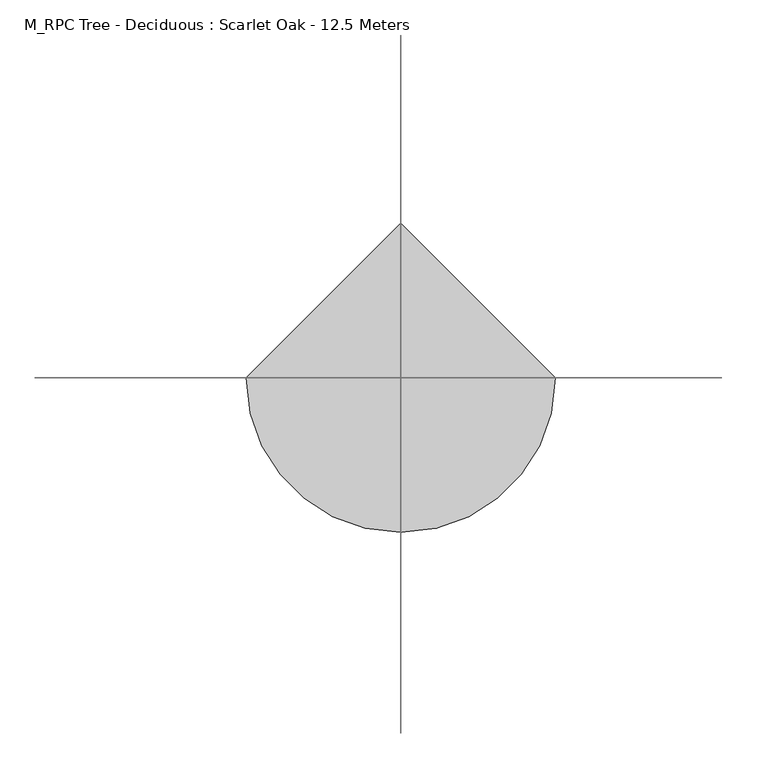
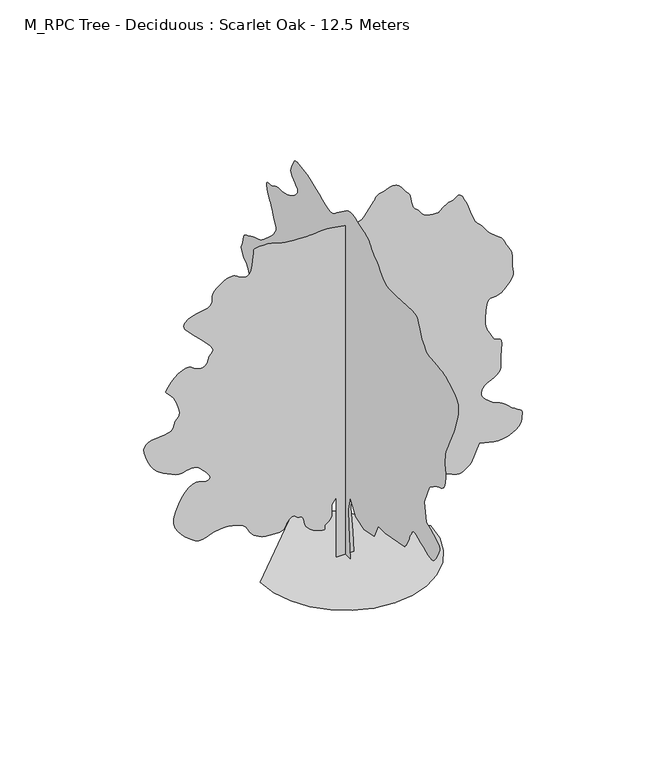
"""IFC4 building model written with IfcOpenShell, lengths in millimetres: geographic element geometry, M_RPC Tree - Deciduous : Scarlet Oak - 12.5 Meters."""

import ifcopenshell
import ifcopenshell.guid

model = None  # the IFC model being written
_history = None  # IfcOwnerHistory: only IFC2X3 demands one
_inside = {}  # id of a spatial element -> (the spatial element, [elements in it])
_under = {}  # id of a project, library or spatial element -> (it, [spatial elements below it])
_declared = {}  # id of a project -> (the project, [libraries it declares])
_typed = {}  # id of a type object -> (the type object, [elements of that type])
_made_of = {}  # id of a material, layer set ... -> (it, [elements and type objects made of it])


def new_model(schema):
    """Start an empty IFC model of exactly this schema.

    Asked for "IFC4X3", IfcOpenShell would pick the latest addendum, in which some entities
    have other attributes; the version numbers below select the first issue.
    IFC2X3 requires an IfcOwnerHistory on every rooted entity: one is made here for all.
    """
    global model, _history
    if schema == "IFC4X3":
        model = ifcopenshell.file(schema_version=(4, 3, 0, 0))
    else:
        model = ifcopenshell.file(schema=schema)
    _inside.clear()
    _under.clear()
    _declared.clear()
    _typed.clear()
    _made_of.clear()
    _history = None
    if model.schema == "IFC2X3":
        org = make("IfcOrganization", Name="unknown")
        user = make(
            "IfcPersonAndOrganization",
            ThePerson=make("IfcPerson", FamilyName="unknown"),
            TheOrganization=org,
        )
        app = make(
            "IfcApplication",
            ApplicationDeveloper=org,
            Version="unknown",
            ApplicationFullName="unknown",
            ApplicationIdentifier="unknown",
        )
        _history = make(
            "IfcOwnerHistory",
            OwningUser=user,
            OwningApplication=app,
            ChangeAction="ADDED",
            CreationDate=0,
        )
    return model


def make(cls, **values):
    """One entity of the class cls with the attributes given. An attribute that is None is left unset."""
    return model.create_entity(
        cls, **{name: value for name, value in values.items() if value is not None}
    )


def rooted(cls, **values):
    """An entity with a GlobalId (a new one), such as an element, a storey or a relation."""
    return make(cls, GlobalId=ifcopenshell.guid.new(), OwnerHistory=_history, **values)


def si_unit(unit_type, name, prefix=None):
    """IfcSIUnit, for example si_unit("LENGTHUNIT", "METRE", prefix="MILLI")."""
    return make("IfcSIUnit", UnitType=unit_type, Prefix=prefix, Name=name)


def assignment(units):
    """IfcUnitAssignment: the units of a project."""
    return None if units is None else make("IfcUnitAssignment", Units=units)


def point(xyz):
    """IfcCartesianPoint."""
    return None if xyz is None else make("IfcCartesianPoint", Coordinates=xyz)


def direction(xyz):
    """IfcDirection."""
    return None if xyz is None else make("IfcDirection", DirectionRatios=xyz)


def frame(location, z_axis=None, x_axis=None):
    """IfcAxis2Placement3D, a coordinate frame: its origin and axes. An axis left out is left unset."""
    return make(
        "IfcAxis2Placement3D",
        Location=point(location),
        Axis=direction(z_axis),
        RefDirection=direction(x_axis),
    )


def origin():
    """The frame at (0, 0, 0) with its axes left unset."""
    return frame((0.0, 0.0, 0.0))


def place(relative_to, where):
    """IfcLocalPlacement: puts the frame where relative to a parent placement (None: the world)."""
    return make(
        "IfcLocalPlacement", PlacementRelTo=relative_to, RelativePlacement=where
    )


def context(
    kind, dimensions, precision=None, world=None, true_north=None, identifier=None
):
    """IfcGeometricRepresentationContext, for example the 3D "Model" context."""
    return make(
        "IfcGeometricRepresentationContext",
        ContextIdentifier=identifier,
        ContextType=kind,
        CoordinateSpaceDimension=dimensions,
        Precision=precision,
        WorldCoordinateSystem=world,
        TrueNorth=true_north,
    )


def project(units=None, contexts=None):
    """IfcProject with its units and contexts."""
    return rooted(
        "IfcProject",
        Name="project",
        RepresentationContexts=contexts,
        UnitsInContext=assignment(units),
    )


def spatial(cls, under=None, at=None, **own):
    """A site, building, storey or space (cls), placed at a placement, below another one or the project."""
    s = rooted(cls, ObjectPlacement=at, **own)
    if under is not None:
        _under.setdefault(under.id(), (under, []))[1].append(s)
    return s


def point_list(points):
    """IfcCartesianPointList2D or 3D."""
    cls = (
        "IfcCartesianPointList2D" if len(points[0]) == 2 else "IfcCartesianPointList3D"
    )
    return make(cls, CoordList=points)


def triangles(points, corners, closed=None, point_numbers=None):
    """IfcTriangulatedFaceSet: each triangle names its three corners, points numbered from 1."""
    return make(
        "IfcTriangulatedFaceSet",
        Coordinates=point_list(points),
        Closed=closed,
        CoordIndex=corners,
        PnIndex=point_numbers,
    )


def shape(context_of_items, identifier, shape_type, items):
    """IfcShapeRepresentation: the items that make up one representation, for example the "Body"."""
    return make(
        "IfcShapeRepresentation",
        ContextOfItems=context_of_items,
        RepresentationIdentifier=identifier,
        RepresentationType=shape_type,
        Items=items,
    )


def source(mapping_origin, context_of_items, identifier, shape_type, items):
    """IfcRepresentationMap: a shape defined once, which mapped items show again and again."""
    return make(
        "IfcRepresentationMap",
        MappingOrigin=mapping_origin,
        MappedRepresentation=shape(context_of_items, identifier, shape_type, items),
    )


def transform(
    local_origin,
    x_axis=None,
    y_axis=None,
    z_axis=None,
    scale=None,
    scale2=None,
    scale3=None,
    uniform=True,
):
    """IfcCartesianTransformationOperator3D, or its non-uniform kind. x_axis, y_axis, z_axis: its Axis1, 2, 3."""
    if uniform:
        return make(
            "IfcCartesianTransformationOperator3D",
            Axis1=direction(x_axis),
            Axis2=direction(y_axis),
            LocalOrigin=point(local_origin),
            Scale=scale,
            Axis3=direction(z_axis),
        )
    return make(
        "IfcCartesianTransformationOperator3DnonUniform",
        Axis1=direction(x_axis),
        Axis2=direction(y_axis),
        LocalOrigin=point(local_origin),
        Scale=scale,
        Axis3=direction(z_axis),
        Scale2=scale2,
        Scale3=scale3,
    )


def mapped(mapping_source, mapping_target):
    """IfcMappedItem: shows the shape of a source again, moved by a transform."""
    return make(
        "IfcMappedItem", MappingSource=mapping_source, MappingTarget=mapping_target
    )


def made_of(thing, what):
    """Note that an element or type object is made of a material, layer set ...; save() writes the relation."""
    if what is not None:
        _made_of.setdefault(what.id(), (what, []))[1].append(thing)
    return thing


def element(
    cls,
    number,
    at=None,
    inside=None,
    cuts=None,
    type_object=None,
    material=None,
    context=None,
    identifier="Body",
    shape_type=None,
    held_by="IfcProductDefinitionShape",
    body=None,
    shapes=None,
    **own,
):
    """One element of the class cls, such as IfcWall. Its Tag is "e" and its number.

    at: its placement. inside: the storey or other place that contains it. cuts: it is an
    opening in that element (IfcRelVoidsElement). A single representation is given by context,
    identifier, shape_type and body (its items); several are given by shapes. held_by: the class
    of the entity that holds the representations. save() writes the other relations.
    """
    e = rooted(cls, Tag="e%d" % number, ObjectPlacement=at, **own)
    if body is not None:
        shapes = [shape(context, identifier, shape_type, body)]
    if shapes is not None:
        e.Representation = make(held_by, Representations=shapes)
    if inside is not None:
        _inside.setdefault(inside.id(), (inside, []))[1].append(e)
    if cuts is not None:
        rooted(
            "IfcRelVoidsElement", RelatingBuildingElement=cuts, RelatedOpeningElement=e
        )
    if type_object is not None:
        _typed.setdefault(type_object.id(), (type_object, []))[1].append(e)
    return made_of(e, material)


def aggregate(whole, parts):
    """IfcRelAggregates: a whole, such as a stair, and the parts it consists of."""
    return rooted("IfcRelAggregates", RelatingObject=whole, RelatedObjects=parts)


def save(model, path):
    """Write the relations noted so far, then the file.

    IfcRelAggregates (storeys below a building ...), IfcRelContainedInSpatialStructure (elements
    in a storey), IfcRelDefinesByType, IfcRelAssociatesMaterial and IfcRelDeclares: one each for
    every whole, place, type object, material and project.
    """
    for whole, parts in _under.values():
        aggregate(whole, parts)
    for where, things in _inside.values():
        rooted(
            "IfcRelContainedInSpatialStructure",
            RelatedElements=things,
            RelatingStructure=where,
        )
    for kind, things in _typed.values():
        rooted("IfcRelDefinesByType", RelatedObjects=things, RelatingType=kind)
    for what, things in _made_of.values():
        rooted("IfcRelAssociatesMaterial", RelatedObjects=things, RelatingMaterial=what)
    for by, libraries in _declared.values():
        rooted("IfcRelDeclares", RelatingContext=by, RelatedDefinitions=libraries)
    model.write(path)


def m_rpc_tree_deciduous_scarlet_oak_12_5_meters_13b38d7d(model_context):
    return source(origin(), model_context, "Body", "Tessellation", [
        triangles([(0.0172504, 306.0074844, 0.0), (0.0172504, -293.5650026, 0.0), (0.0172504, -196.8600042, 1141.1199549), (0.0172504, -177.5184886, 1682.6674953), (0.0172504, -293.5650026, 2185.5349113), (0.0172504, -603.0224945, 1682.6674953), (0.0172504, -1105.8875124, 1527.9400211), (0.0172504, -1686.1174301, 1663.3275421), (0.0172504, -1918.2099495, 2146.8525341), (0.0172504, -2324.3725124, 2146.8525341), (0.0172504, -3446.1498253, 2359.6049549), (0.0172504, -3487.4249222, 2409.394939), (0.0172504, -3527.7000801, 2459.5225479), (0.0172504, -3565.9250725, 2510.3249702), (0.0172504, -3601.0999603, 2562.1500046), (0.0172504, -3632.2248047, 2615.3249565), (0.0172504, -3658.2749588, 2670.2000954), (0.0172504, -3678.2499023, 2727.0748215), (0.0172504, -3697.649881, 2785.6750237), (0.0172504, -3722.1248405, 2845.2748741), (0.0172504, -3750.8248329, 2905.7249634), (0.0172504, -3782.89991, 2966.8500114), (0.0172504, -3817.5248314, 3028.475029), (0.0172504, -3853.8249413, 3090.4500252), (0.0172504, -3890.9999977, 3152.5750122), (0.0172504, -3908.7000801, 3172.6499496), (0.0172504, -3933.1750397, 3188.8498329), (0.0172504, -3971.1750458, 3197.2499016), (0.0172504, -4029.4749756, 3193.9748108), (0.0172504, -4114.8499969, 3175.1500877), (0.0172504, -4234.0499886, 3136.8498093), (0.0172504, -4393.8498276, 3075.2250824), (0.0172504, -4562.5749939, 3002.6998581), (0.0172504, -4706.2499451, 2937.9750298), (0.0172504, -4828.2750549, 2886.4249786), (0.0172504, -4932.0251175, 2853.4999535), (0.0172504, -5020.8999252, 2844.5999153), (0.0172504, -5098.249855, 2865.1248253), (0.0172504, -5167.4996979, 2920.4999336), (0.0172504, -5237.3750839, 3007.7248421), (0.0172504, -5309.5997452, 3113.9000473), (0.0172504, -5377.0996948, 3229.5499649), (0.0172504, -5432.7497864, 3345.1998825), (0.0172504, -5469.4498718, 3451.3750877), (0.0172504, -5480.1248016, 3538.6249947), (0.0172504, -5457.6250122, 3597.424894), (0.0172504, -5402.6498795, 3641.6998077), (0.0172504, -5323.3000717, 3691.0249947), (0.0172504, -5223.6747574, 3744.5999222), (0.0172504, -5107.774855, 3801.5499344), (0.0172504, -4979.7251129, 3861.0500816), (0.0172504, -4843.5499947, 3922.224836), (0.0172504, -4703.3248329, 3984.2498291), (0.0172504, -4587.2749397, 4641.8498062), (0.0172504, -4877.3749649, 5318.7747665), (0.0172504, -4886.5249878, 5331.7001404), (0.0172504, -4900.7247025, 5347.4747589), (0.0172504, -4925.0999588, 5369.0251877), (0.0172504, -4964.6748688, 5399.20009), (0.0172504, -5024.5497025, 5440.8498734), (0.0172504, -5109.8247299, 5496.8999405), (0.0172504, -5225.5246445, 5570.225116), (0.0172504, -5351.0501221, 5636.6501312), (0.0172504, -5462.3497238, 5680.0498077), (0.0172504, -5559.4501923, 5715.3499786), (0.0172504, -5642.3497833, 5757.424736), (0.0172504, -5711.0246613, 5821.1499161), (0.0172504, -5765.4998245, 5921.4001923), (0.0172504, -5805.7496933, 6073.0746552), (0.0172504, -5829.0500153, 6222.0498642), (0.0172504, -5835.7501877, 6317.5748474), (0.0172504, -5830.6249191, 6379.6001312), (0.0172504, -5818.3750854, 6428.1000778), (0.0172504, -5803.7748138, 6483.0246323), (0.0172504, -5791.5499786, 6564.3249023), (0.0172504, -5786.4247101, 6691.9996674), (0.0172504, -5788.2251816, 6832.849791), (0.0172504, -5796.1246994, 6949.6746368), (0.0172504, -5813.8247818, 7056.3751007), (0.0172504, -5845.0496201, 7166.7747574), (0.0172504, -5893.550148, 7294.7750839), (0.0172504, -5963.0249771, 7454.2496521), (0.0172504, -6057.1750443, 7659.049942), (0.0172504, -6146.5748199, 7844.1746887), (0.0172504, -6206.1746704, 7955.8748474), (0.0172504, -6246.4751175, 8024.9497009), (0.0172504, -6277.9999374, 8082.1746964), (0.0172504, -6311.2246536, 8158.3496979), (0.0172504, -6356.599791, 8284.2751511), (0.0172504, -6424.6747055, 8490.6997604), (0.0172504, -6498.0248795, 8729.4997192), (0.0172504, -6547.3747742, 8935.1499573), (0.0172504, -6565.2498459, 9112.3746048), (0.0172504, -6544.199968, 9265.925116), (0.0172504, -6476.8250107, 9400.5250397), (0.0172504, -6355.6498489, 9520.8996689), (0.0172504, -6173.2249374, 9631.8248749), (0.0172504, -5996.2246948, 9723.0001236), (0.0172504, -5879.7998245, 9785.7747803), (0.0172504, -5799.2250916, 9827.2001587), (0.0172504, -5729.799678, 9854.4496582), (0.0172504, -5646.85009, 9874.575174), (0.0172504, -5525.6749283, 9894.699527), (0.0172504, -5341.575119, 9921.9501892), (0.0172504, -5144.0999634, 9943.4244598), (0.0172504, -4990.9500092, 9951.725116), (0.0172504, -4869.5998581, 9962.0244873), (0.0172504, -4767.5499825, 9989.5995483), (0.0172504, -4672.2499855, 10049.6493713), (0.0172504, -4571.2000488, 10157.425351), (0.0172504, -4451.8750648, 10328.0998169), (0.0172504, -4347.6750298, 10515.7499908), (0.0172504, -4286.1000092, 10666.5500885), (0.0172504, -4245.8498497, 10783.8243256), (0.0172504, -4205.5749825, 10871.0003998), (0.0172504, -4143.9999619, 10931.4501984), (0.0172504, -4039.7999268, 10968.5502594), (0.0172504, -3871.650016, 10985.7003754), (0.0172504, -2943.2749969, 10927.6748474), (0.0172504, -2772.1499771, 10930.6746643), (0.0172504, -2632.8250511, 10930.2746887), (0.0172504, -2514.4500092, 10937.3242584), (0.0172504, -2406.244986, 10962.6250397), (0.0172504, -2297.3599171, 11017.0496246), (0.0172504, -2176.9724979, 11111.3752625), (0.0172504, -2034.2549011, 11256.4745453), (0.0172504, -1896.7275398, 11403.0249023), (0.0172504, -1793.7049038, 11502.8746216), (0.0172504, -1717.0749882, 11568.5752625), (0.0172504, -1658.7124168, 11612.6248993), (0.0172504, -1610.5024235, 11647.5250946), (0.0172504, -1564.3199226, 11685.7995026), (0.0172504, -1512.0500027, 11739.9996826), (0.0172504, -1461.8649845, 11803.9992645), (0.0172504, -1420.8125484, 11863.6002777), (0.0172504, -1379.087479, 11919.1503754), (0.0172504, -1326.8724976, 11970.9495392), (0.0172504, -1254.3574471, 12019.4000702), (0.0172504, -1151.7299904, 12064.7996246), (0.0172504, -1009.182514, 12107.4749268), (0.0172504, -849.1549999, 12154.4999634), (0.0172504, -699.9524792, 12206.6002716), (0.0172504, -560.5600064, 12254.6496643), (0.0172504, -429.9675053, 12289.4998627), (0.0172504, -307.1549798, 12302.0246796), (0.0172504, -191.1079934, 12283.0746735), (0.0172504, -80.8134993, 12223.5248199), (0.0172504, 499.4174812, 11798.0252106), (0.0172504, 562.2325061, 11740.8496307), (0.0172504, 623.0199657, 11688.7493225), (0.0172504, 689.217524, 11646.7751404), (0.0172504, 768.2749804, 11620.0500275), (0.0172504, 867.6299623, 11613.6248383), (0.0172504, 994.7275097, 11632.5748444), (0.0172504, 1157.0125168, 11681.9753174), (0.0172504, 1341.1749676, 11755.3243286), (0.0172504, 1526.6899521, 11837.8251068), (0.0172504, 1710.1749733, 11922.0246185), (0.0172504, 1888.2475342, 12000.4500641), (0.0172504, 2057.5249924, 12065.6995697), (0.0172504, 2214.6199093, 12110.3003357), (0.0172504, 2356.1550201, 12126.8249084), (0.0172504, 2484.8875694, 12135.849939), (0.0172504, 2604.4750374, 12156.3742676), (0.0172504, 2712.9248131, 12178.575238), (0.0172504, 2808.1498146, 12192.6743774), (0.0172504, 2888.1748718, 12188.8501923), (0.0172504, 2950.9248207, 12157.2753754), (0.0172504, 2994.400074, 12088.1249451), (0.0172504, 3033.2500282, 12001.2500153), (0.0172504, 3077.8499222, 11921.1246735), (0.0172504, 3119.7499809, 11845.0502472), (0.0172504, 3150.4998482, 11770.3245758), (0.0172504, 3161.6000427, 11694.2745667), (0.0172504, 3144.6249161, 11614.1503876), (0.0172504, 3091.124984, 11527.2498779), (0.0172504, 3009.2500397, 11447.6245056), (0.0172504, 2921.5998665, 11385.2492432), (0.0172504, 2841.4248184, 11331.3502075), (0.0172504, 2781.8749649, 11277.1000305), (0.0172504, 2756.1750801, 11213.7248291), (0.0172504, 2777.4749428, 11132.4251404), (0.0172504, 2859.0249069, 11024.3747589), (0.0172504, 2971.6250107, 10916.724353), (0.0172504, 3077.7999252, 10838.2000763), (0.0172504, 3178.2249001, 10782.3), (0.0172504, 3273.574894, 10742.6745117), (0.0172504, 3364.5248657, 10712.8251709), (0.0172504, 3451.7750633, 10686.4000397), (0.0172504, 3535.9498672, 10656.8995148), (0.0172504, 3620.024968, 10634.1753204), (0.0172504, 3706.4749237, 10626.6746155), (0.0172504, 3795.2750267, 10625.9502411), (0.0172504, 3886.4499847, 10623.5248077), (0.0172504, 3979.9997978, 10610.9499939), (0.0172504, 4075.9250473, 10579.7495728), (0.0172504, 4174.1998627, 10521.5252197), (0.0172504, 4275.775058, 10469.7993073), (0.0172504, 4375.6250679, 10451.2492767), (0.0172504, 4464.9998451, 10446.8995422), (0.0172504, 4535.0999268, 10437.8245148), (0.0172504, 4577.0999794, 10405.075351), (0.0172504, 4582.2249573, 10329.6753021), (0.0172504, 4541.6998146, 10192.7243591), (0.0172504, 4481.7999825, 10048.5994354), (0.0172504, 4432.0748199, 9951.4995483), (0.0172504, 4388.424868, 9882.1247131), (0.0172504, 4346.824791, 9821.224942), (0.0172504, 4303.174839, 9749.4996689), (0.0172504, 4253.4249687, 9647.6750702), (0.0172504, 4193.5498444, 9496.4499985), (0.0172504, 4130.2749275, 9347.6997757), (0.0172504, 4075.8250534, 9253.7496964), (0.0172504, 4034.1999779, 9195.999733), (0.0172504, 4009.500032, 9155.8498581), (0.0172504, 4005.7749687, 9114.7000443), (0.0172504, 4027.0998299, 9053.8996857), (0.0172504, 4077.4999512, 8954.8999146), (0.0172504, 4167.2249977, 8823.6747849), (0.0172504, 4293.1248711, 8684.3501495), (0.0172504, 4439.3499573, 8545.349913), (0.0172504, 4589.9500671, 8415.1497208), (0.0172504, 4729.0750053, 8302.1996384), (0.0172504, 4840.7748734, 8214.9747299), (0.0172504, 4909.1747681, 8161.9000626), (0.0172504, 4969.9001312, 8128.6997635), (0.0172504, 5061.0747986, 8095.1500671), (0.0172504, 5170.5250946, 8060.9248306), (0.0172504, 5286.0750183, 8025.6746567), (0.0172504, 5395.524733, 7989.0751465), (0.0172504, 5486.6999817, 7950.8001572), (0.0172504, 5547.4247635, 7910.4747116), (0.0172504, 5598.275148, 7876.9750122), (0.0172504, 5663.0246841, 7853.2997131), (0.0172504, 5734.1749924, 7830.2999542), (0.0172504, 5804.3247803, 7798.8251312), (0.0172504, 5866.0250839, 7749.7746368), (0.0172504, 5911.8001968, 7673.9746124), (0.0172504, 5934.2499893, 7562.325032), (0.0172504, 5952.6250305, 7450.1749008), (0.0172504, 5984.1998474, 7370.8500916), (0.0172504, 6018.4750809, 7312.1496048), (0.0172504, 6044.9996246, 7261.899765), (0.0172504, 6053.224704, 7207.9501511), (0.0172504, 6032.699794, 7138.074765), (0.0172504, 5972.9249542, 7040.1249298), (0.0172504, 5898.7248322, 6948.3747162), (0.0172504, 5838.7250061, 6893.5251572), (0.0172504, 5788.2001831, 6857.9500031), (0.0172504, 5742.4000717, 6824.0497467), (0.0172504, 5696.6249588, 6774.2498795), (0.0172504, 5646.1001358, 6690.9747299), (0.0172504, 5586.0997284, 6556.5997925), (0.0172504, 5520.6996506, 6421.9998688), (0.0172504, 5460.6998245, 6337.1498154), (0.0172504, 5411.5249191, 6283.0746277), (0.0172504, 5378.6001846, 6240.824881), (0.0172504, 5367.3247101, 6191.4999847), (0.0172504, 5383.09991, 6116.0999359), (0.0172504, 5431.3748703, 5995.7247253), (0.0172504, 5495.5000259, 5864.0496231), (0.0172504, 5555.8748291, 5761.8250488), (0.0172504, 5613.5747955, 5680.5747757), (0.0172504, 5669.5498672, 5611.8249023), (0.0172504, 5724.8749786, 5547.1497803), (0.0172504, 5780.5250702, 5478.0749268), (0.0172504, 5837.5250793, 5396.1496948), (0.0172504, 5903.6751114, 5315.3499756), (0.0172504, 5980.6500641, 5249.4249298), (0.0172504, 6060.324852, 5189.6000931), (0.0172504, 6134.5999695, 5127.0498413), (0.0172504, 6195.3247513, 5053.0247086), (0.0172504, 6234.3996918, 4958.6746536), (0.0172504, 6243.6997055, 4835.2499199), (0.0172504, 6251.5248093, 4738.3250221), (0.0172504, 6280.349794, 4706.349939), (0.0172504, 6313.2251129, 4704.825032), (0.0172504, 6333.2500534, 4699.249791), (0.0172504, 6323.4750687, 4655.0998695), (0.0172504, 6267.0500244, 4537.8750481), (0.0172504, 6146.999794, 4313.0498177), (0.0172504, 6021.4748978, 4060.8748032), (0.0172504, 5945.6998718, 3875.3750793), (0.0172504, 5898.3248566, 3742.6250427), (0.0172504, 5858.0749878, 3648.7999557), (0.0172504, 5803.5998245, 3580.0000854), (0.0172504, 5713.6000854, 3522.3748238), (0.0172504, 5566.7747452, 3462.0500175), (0.0172504, 5397.2496277, 3413.0998077), (0.0172504, 5248.0500137, 3392.5748978), (0.0172504, 5111.0246567, 3390.9999939), (0.0172504, 4978.0746323, 3398.8998024), (0.0172504, 4841.0498566, 3406.7749031), (0.0172504, 4691.8499519, 3405.1999992), (0.0172504, 4522.3498329, 3384.6750893), (0.0172504, 4353.2999771, 3366.3000481), (0.0172504, 4207.2498802, 3370.249807), (0.0172504, 4078.7998718, 3385.7000267), (0.0172504, 3962.5249924, 3401.8249146), (0.0172504, 3853.0249901, 3407.7998405), (0.0172504, 3744.8749054, 3392.799884), (0.0172504, 3632.6500694, 3345.9998337), (0.0172504, 3525.249939, 3296.2499634), (0.0172504, 3436.4248375, 3270.1998093), (0.0172504, 3368.249929, 3253.6249489), (0.0172504, 3322.75009, 3232.3250862), (0.0172504, 3301.9499062, 3192.0499283), (0.0172504, 3307.8748352, 3118.6500481), (0.0172504, 3342.5500443, 2997.8498634), (0.0172504, 3398.4748283, 2869.5248474), (0.0172504, 3465.5748024, 2778.7248665), (0.0172504, 3542.0000793, 2719.2500084), (0.0172504, 3625.8499031, 2684.8000763), (0.0172504, 3715.274968, 2669.1248703), (0.0172504, 3808.4248055, 2665.9500641), (0.0172504, 3903.4248207, 2669.0498749), (0.0172504, 4270.9250633, 2262.8999565), (0.0172504, 4299.7250496, 2217.1674282), (0.0172504, 4327.3498169, 2170.5925095), (0.0172504, 4352.6250183, 2122.3249615), (0.0172504, 4374.3248566, 2071.5174522), (0.0172504, 4391.2999832, 2017.3299168), (0.0172504, 4402.3498901, 1958.9124069), (0.0172504, 4406.2999397, 1895.4199162), (0.0172504, 4405.6249809, 1829.2200325), (0.0172504, 4400.8999786, 1763.6974331), (0.0172504, 4388.0248924, 1699.5299835), (0.0172504, 4362.9999664, 1637.3900265), (0.0172504, 4321.7248695, 1577.9574623), (0.0172504, 4260.1498489, 1521.9075405), (0.0172504, 4174.1998627, 1469.9175453), (0.0172504, 4092.2249245, 1425.7650078), (0.0172504, 4034.5999535, 1391.4249527), (0.0172504, 3985.4250481, 1364.8674168), (0.0172504, 3928.800016, 1344.0599659), (0.0172504, 3848.8499542, 1326.9749622), (0.0172504, 3729.6499626, 1311.5799717), (0.0172504, 3555.2998489, 1295.8475018), (0.0172504, 3356.9750359, 1298.1024513), (0.0172504, 3174.2248535, 1332.8375404), (0.0172504, 3003.6500908, 1392.27243), (0.0172504, 2841.8750816, 1468.6199501), (0.0172504, 2685.525032, 1554.1049938), (0.0172504, 2531.1748604, 1640.9424259), (0.0172504, 2375.4949734, 1721.3500179), (0.0172504, 2236.6674007, 1794.4849434), (0.0172504, 2129.3049133, 1863.5599422), (0.0172504, 2044.6099377, 1926.8850014), (0.0172504, 1973.7875164, 1982.7650208), (0.0172504, 1908.0399307, 2029.5099873), (0.0172504, 1838.5700432, 2065.4300331), (0.0172504, 1756.5824604, 2088.8299129), (0.0172504, 1666.4174698, 2108.5649002), (0.0172504, 1577.6074837, 2133.0375343), (0.0172504, 1489.134977, 2159.8799366), (0.0172504, 1399.9875114, 2186.7200134), (0.0172504, 1309.1449459, 2211.1925022), (0.0172504, 1215.5974583, 2230.9274895), (0.0172504, 1118.3299942, 2243.5575325), (0.0172504, 1018.8625191, 2250.1549496), (0.0172504, 919.3925005, 2253.7074944), (0.0172504, 819.9249527, 2254.7224033), (0.0172504, 720.4574776, 2253.7074944), (0.0172504, 620.9900024, 2251.1700039), (0.0172504, 521.5199839, 2247.6174591), (0.0172504, 422.0525087, 2243.5575325), (0.0172504, 228.6430025, 1953.4425373), (0.0172504, 189.960498, 1508.5999226), (280.4450004, 0.0006008, 0.0092122), (-299.78499, 0.0006008, 0.0092122), (-299.78499, 0.0004756, 2127.5199932), (-454.5149895, 0.0004756, 1914.7698978), (-454.5149895, 0.0005007, 1682.6775238), (-450.962481, 0.0005007, 1628.8274677), (-450.962481, 0.0005007, 1575.1449886), (-458.0674979, 0.0005007, 1521.8024597), (-475.8274967, 0.0005257, 1468.967458), (-507.8000001, 0.0005257, 1416.8100311), (-557.5350094, 0.0005257, 1365.4949947), (-628.5824896, 0.0005257, 1315.1974834), (-684.2375227, 0.0005257, 1262.982502), (-699.6325132, 0.0005257, 1210.0899456), (-696.0799685, 0.0005257, 1162.9524885), (-694.8950117, 0.0005257, 1127.990015), (-717.3950191, 0.0005257, 1111.6374521), (-784.8899546, 0.0005257, 1120.3224598), (-918.6974848, 0.0005257, 1160.4700092), (-1071.3399845, 0.0005257, 1223.0050003), (-1185.4124548, 0.0005257, 1293.6575191), (-1267.3424103, 0.0005257, 1371.0799736), (-1323.5625252, 0.0005257, 1453.9124176), (-1360.49748, 0.0005007, 1540.8049335), (-1384.5749348, 0.0005007, 1630.4049877), (-1402.2250202, 0.0005007, 1721.359901), (-1406.7349194, 0.0005007, 1746.1124599), (-1413.4449749, 0.0005007, 1770.1899147), (-1424.5524364, 0.0005007, 1792.9174519), (-1442.2599312, 0.0005007, 1813.6099388), (-1468.7599125, 0.0005007, 1831.5975037), (-1506.2599491, 0.0005007, 1846.2024261), (-1556.9524944, 0.0005007, 1856.747422), (-1607.6450397, 0.0005007, 1874.1124958), (-1647.509903, 0.0005007, 1903.3224861), (-1682.3024014, 0.0004756, 1934.8999191), (-1717.7700039, 0.0004756, 1959.3724079), (-1759.6674465, 0.0004756, 1967.2674202), (-1813.7424889, 0.0004756, 1949.1099529), (-1885.7500122, 0.0005007, 1895.4274738), (-1949.0724552, 0.0005007, 1820.3199944), (-1984.9925011, 0.0005007, 1746.902528), (-2011.0999191, 0.0005007, 1679.2374722), (-2044.9875309, 0.0005007, 1621.382428), (-2104.2525181, 0.0005007, 1577.402409), (-2206.4824699, 0.0005007, 1551.3499294), (-2369.2750042, 0.0005007, 1547.2900028), (-2549.149926, 0.0005007, 1559.2449417), (-2695.2000229, 0.0005007, 1578.979929), (-2813.8250496, 0.0005007, 1607.1750103), (-2911.4999016, 0.0005007, 1644.5025284), (-2994.6250603, 0.0005007, 1691.6425289), (-3069.5998444, 0.0005007, 1749.2724415), (-3142.9250198, 0.0005007, 1818.0648994), (-3205.1000038, 0.0005007, 1893.5100037), (-3249.7248962, 0.0004756, 1969.2975288), (-3287.549913, 0.0004756, 2043.389954), (-3329.4499718, 0.0004756, 2113.7624027), (-3386.2249947, 0.0004756, 2178.3824409), (-3468.7249008, 0.0004756, 2235.2224308), (-3587.7499031, 0.0004756, 2282.2499382), (-3707.4248657, 0.0004756, 2317.9974655), (-3794.2497986, 0.0004506, 2343.2600224), (-3862.8249733, 0.0004506, 2359.3875263), (-3927.674794, 0.0004506, 2367.7325111), (-4003.3248276, 0.0004506, 2369.6499813), (-4104.3750549, 0.0004506, 2366.4924706), (-4245.3498802, 0.0004506, 2359.6125126), (-4400.3500122, 0.0004506, 2335.1974331), (-4538.1250328, 0.0004756, 2289.8050003), (-4665.0498436, 0.0004756, 2240.3524956), (-4787.5749229, 0.0004756, 2203.7574909), (-4912.1501678, 0.0004756, 2196.9349422), (-5045.1501892, 0.0004756, 2236.7999508), (-5193.0498825, 0.0004506, 2340.272414), (-5347.7997391, 0.0004506, 2478.6475433), (-5490.6747391, 0.0004506, 2615.9999153), (-5612.2498764, 0.0004256, 2758.4499413), (-5703.0251495, 0.0004256, 2912.049868), (-5753.5499725, 0.0004256, 3082.8999046), (-5754.3499237, 0.0004005, 3277.0999695), (-5695.9250015, 0.0004005, 3500.7249825), (-5598.1501556, 0.0003755, 3726.2748779), (-5489.1998291, 0.0003755, 3919.6999901), (-5372.1499969, 0.0003505, 4077.2499664), (-5250.0248932, 0.0003505, 4195.2000343), (-5125.8499146, 0.0003505, 4269.8498383), (-5002.6998734, 0.0003505, 4297.4998947), (-4883.6001663, 0.0003505, 4274.3748528), (-4771.2750458, 0.0003505, 4235.4749016), (-4671.8250114, 0.0003505, 4218.8750427), (-4593.3248611, 0.0003505, 4225.6499199), (-4543.9249695, 0.0003505, 4256.7750549), (-4531.7498405, 0.0003505, 4313.2748039), (-4564.899852, 0.0003505, 4396.1749763), (-4651.4997986, 0.0003254, 4506.4749298), (-4752.500029, 0.0003254, 4617.0998634), (-4829.4749817, 0.0003254, 4702.3498924), (-4891.5496811, 0.0003254, 4765.2748306), (-4947.8747314, 0.0003254, 4808.9247826), (-5007.6001556, 0.0003254, 4836.3248543), (-5079.8248169, 0.0003004, 4850.5498581), (-5173.7248993, 0.0003004, 4854.5999016), (-5270.0248352, 0.0003254, 4845.5248741), (-5349.7751999, 0.0003254, 4824.5999886), (-5422.3998367, 0.0003254, 4801.3249557), (-5497.39991, 0.0003254, 4785.1247818), (-5584.2248428, 0.0003254, 4785.5250481), (-5692.3746368, 0.0003254, 4811.9748871), (-5831.3248764, 0.0003004, 4873.9498833), (-5978.7751785, 0.0003004, 4948.0997177), (-6108.6248108, 0.0003004, 5012.4248611), (-6224.624707, 0.0003004, 5078.4748993), (-6330.4496429, 0.0003004, 5157.6997147), (-6429.8749695, 0.0003004, 5261.5997681), (-6526.574881, 0.0002754, 5401.7249359), (-6624.2997299, 0.0002754, 5589.5750977), (-6705.1000305, 0.0002503, 5784.4998276), (-6749.6996338, 0.0002503, 5941.2001465), (-6759.8001801, 0.0002503, 6064.0746231), (-6737.074823, 0.0002253, 6157.4997345), (-6683.2246216, 0.0002253, 6225.8996292), (-6599.9500534, 0.0002253, 6273.6496216), (-6488.899855, 0.0002253, 6305.1750229), (-6357.7997177, 0.0002253, 6323.2750809), (-6219.2750336, 0.0002253, 6333.9500107), (-6082.3996674, 0.0002253, 6346.2748398), (-5956.3748016, 0.0002253, 6369.4501694), (-5850.3248795, 0.0002253, 6412.5998611), (-5773.3499268, 0.0002253, 6484.8251038), (-5734.5999664, 0.0002003, 6595.2997559), (-5705.9749695, 0.0002003, 6701.9746399), (-5661.749762, 0.0002003, 6771.4500504), (-5614.8497177, 0.0002003, 6825.699646), (-5578.0746368, 0.0002003, 6886.6999924), (-5564.3248947, 0.0001752, 6976.4747452), (-5586.4247086, 0.0001752, 7116.9998886), (-5657.2500366, 0.0001752, 7330.2496628), (-5757.5497284, 0.0001502, 7540.2996323), (-5853.4746872, 0.0001502, 7672.5247009), (-5935.8498917, 0.0001502, 7750.975145), (-5995.5747345, 0.0001252, 7799.6250824), (-6023.4747757, 0.0001252, 7842.5247894), (-6010.4499893, 0.0001252, 7903.7251236), (-5947.3497711, 0.0001252, 8007.1996216), (-5845.6501648, 0.0001252, 8136.3248795), (-5728.0247864, 0.0001001, 8253.9496765), (-5602.2749039, 0.0001001, 8353.3000076), (-5476.1750427, 0.0001001, 8427.6251221), (-5357.5497253, 0.0001001, 8470.1248535), (-5254.1246429, 0.0001001, 8474.0746124), (-5173.7248993, 0.0001001, 8432.6998123), (-5094.9000595, 0.0001001, 8371.00009), (-4997.8001724, 0.0001001, 8322.8501221), (-4892.5751999, 0.0001001, 8294.6500992), (-4789.3748131, 0.0001001, 8292.8496277), (-4698.3748444, 0.0001001, 8323.8750595), (-4629.6999664, 0.0001001, 8394.1248413), (-4593.4998505, 0.0001001, 8510.0497421), (-4560.3248405, 0.0001001, 8620.5749725), (-4508.224823, 7.51e-05, 8686.1000427), (-4458.4999512, 7.51e-05, 8730.2996704), (-4432.4497971, 7.51e-05, 8776.8747345), (-4451.3998032, 7.51e-05, 8849.4999527), (-4536.6498322, 7.51e-05, 8971.8750412), (-4709.5500343, 5.01e-05, 9167.6497192), (-4926.3498825, 5.01e-05, 9388.7995926), (-5120.1496811, 2.5e-05, 9575.0998489), (-5277.4249649, 2.5e-05, 9731.9745758), (-5384.5998184, 2.5e-05, 9864.8246063), (-5428.2000641, 0.0, 9979.0746094), (-5394.6497864, 0.0, 10080.1254181), (-5270.4248108, 0.0, 10173.3743774), (-5104.7500397, 0.0, 10245.2246429), (-4956.3497955, 0.0, 10286.2744629), (-4825.8749107, 0.0, 10308.3742767), (-4714.0000534, -2.5e-05, 10323.3745239), (-4621.3998917, -2.5e-05, 10343.1000641), (-4548.7749641, -2.5e-05, 10379.4245911), (-4496.7749405, -2.5e-05, 10444.1497101), (-4470.8500694, -2.5e-05, 10520.7252686), (-4466.9000198, -2.5e-05, 10587.8246613), (-4471.4000359, -2.5e-05, 10650.1999237), (-4470.8500694, -2.5e-05, 10712.5751862), (-4451.6747864, -5.01e-05, 10779.6745789), (-4400.3500122, -5.01e-05, 10856.2501373), (-4303.3748268, -5.01e-05, 10947.0248291), (-4184.6748047, -5.01e-05, 11036.8495789), (-4076.1250351, -5.01e-05, 11106.7243835), (-3976.0500389, -7.51e-05, 11155.5993073), (-3882.7249214, -7.51e-05, 11182.4999908), (-3794.4750755, -7.51e-05, 11186.3997528), (-3709.6000237, -7.51e-05, 11166.2498199), (-3626.4498665, -5.01e-05, 11121.1002502), (-3540.7248665, -5.01e-05, 11065.9001312), (-3452.3250298, -5.01e-05, 11022.8748505), (-3365.6000908, -5.01e-05, 11001.8249725), (-3284.9500717, -5.01e-05, 11012.5998962), (-3214.7999931, -5.01e-05, 11064.9746063), (-3159.5498772, -7.51e-05, 11168.7996643), (-3123.5750381, -7.51e-05, 11333.8500549), (-3102.0998955, -7.51e-05, 11511.0752838), (-3086.6999634, -0.0001001, 11648.0250641), (-3076.3750122, -0.0001001, 11749.4746857), (-3070.1248123, -0.0001001, 11820.1250244), (-3066.9000092, -0.0001001, 11864.7246277), (-3065.7250809, -0.0001001, 11888.0243683), (-3065.5500916, -0.0001001, 11894.7251221), (-3040.1248993, -0.0001001, 11898.674881), (-2971.0500458, -0.0001001, 11907.37435), (-2869.1498703, -0.0001001, 11916.0494019), (-2745.2748734, -0.0001001, 11920.0003235), (-2610.2249771, -0.0001001, 11914.4750793), (-2474.8323692, -0.0001001, 11894.7251221), (-2349.9349056, -0.0001001, 11856.0495758), (-2235.4099194, -0.0001001, 11813.024295), (-2120.5474537, -0.0001001, 11781.8494537), (-2000.2725277, -0.0001001, 11760.1251984), (-1869.507399, -0.0001001, 11745.5249268), (-1723.1824642, -0.0001001, 11735.6743652), (-1556.2175102, -0.0001001, 11728.174823), (-1363.5400269, -0.0001001, 11720.6752808), (-1177.5749971, -0.0001001, 11719.599765), (-1024.4249702, -0.0001001, 11728.6747925), (-889.5449764, -0.0001001, 11741.475174), (-758.3875025, -0.0001001, 11751.5745575), (-616.4049625, -0.0001001, 11752.5244995), (-449.0450109, -0.0001001, 11737.9253906), (-241.7632409, -0.0001001, 11701.3252991), (-32.2257492, -0.0001001, 11657.8000488), (136.7124946, -0.0001001, 11627.7995544), (271.8174929, -0.0001001, 11613.0248749), (379.8574825, -0.0001001, 11615.1503265), (467.5974758, -0.0001001, 11635.9246399), (541.8025031, -0.0001001, 11676.9744598), (609.2425, -0.0001001, 11739.9996826), (899.3574589, -0.0001252, 12107.4749268), (942.8899761, -0.0001252, 12164.1493744), (977.6249926, -0.0001252, 12217.4496094), (1008.9749685, -0.0001252, 12266.3245331), (1042.3574512, -0.0001252, 12309.7997864), (1083.1825029, -0.0001252, 12346.8498505), (1136.864982, -0.0001252, 12376.4503693), (1208.8149508, -0.0001252, 12397.6002411), (1297.0049892, -0.0001502, 12421.8499237), (1393.3149536, -0.0001502, 12454.2246918), (1494.0224693, -0.0001502, 12483.8752075), (1595.4100307, -0.0001502, 12499.9998047), (1693.7499584, -0.0001502, 12491.7747253), (1785.3224213, -0.0001502, 12448.349469), (1866.4099136, -0.0001252, 12358.9246948), (1938.4149662, -0.0001252, 12256.9251068), (2004.3324543, -0.0001252, 12177.5752991), (2062.8075188, -0.0001252, 12112.7746033), (2112.4850098, -0.0001252, 12054.4246765), (2152.0125389, -0.0001252, 11994.3748535), (2180.0374271, -0.0001001, 11924.5000488), (2195.2049606, -0.0001001, 11836.6995941), (2205.7499565, -0.0001001, 11745.6993347), (2220.3550243, -0.0001001, 11669.9248901), (2238.3424438, -0.0001001, 11606.8252533), (2259.0349308, -7.51e-05, 11553.8749969), (2281.7599972, -7.51e-05, 11508.5242767), (2305.8374519, -7.51e-05, 11468.274408), (2330.5924816, -7.51e-05, 11430.5499664), (2355.6274361, -7.51e-05, 11413.5742584), (2381.6799156, -7.51e-05, 11394.2242767), (2409.760033, -7.51e-05, 11370.1501648), (2440.8873482, -7.51e-05, 11338.9753235), (2476.0724098, -7.51e-05, 11298.3243164), (2516.3248947, -7.51e-05, 11245.8251953), (2562.6749725, -7.51e-05, 11179.1246155), (2631.3748489, -5.01e-05, 11115.7249969), (2728.4750267, -5.01e-05, 11072.3253204), (2839.7749191, -5.01e-05, 11045.1246552), (2951.0748116, -5.01e-05, 11030.4743866), (3048.1749893, -5.01e-05, 11024.6003265), (3116.8748657, -5.01e-05, 11023.8247925), (3142.9250198, -5.01e-05, 11024.4003387), (3156.2750771, -5.01e-05, 11038.3250702), (3192.9998703, -5.01e-05, 11074.2252045), (3247.9750031, -5.01e-05, 11123.3501129), (3316.1499115, -7.51e-05, 11176.8503357), (3392.4249069, -7.51e-05, 11225.9752441), (3471.7750053, -7.51e-05, 11261.8997955), (3549.0749382, -7.51e-05, 11275.824527), (3618.3750687, -7.51e-05, 11292.800235), (3679.549823, -7.51e-05, 11331.0746429), (3736.3498444, -7.51e-05, 11371.7244873), (3792.4499084, -7.51e-05, 11395.8253418), (3851.6000771, -7.51e-05, 11384.3748779), (3917.5248322, -7.51e-05, 11318.4498322), (3993.9248199, -7.51e-05, 11179.1246155), (4065.8750793, -5.01e-05, 11015.4253052), (4119.5500008, -5.01e-05, 10883.1996552), (4160.3748344, -5.01e-05, 10773.6249481), (4193.7498322, -2.5e-05, 10677.9493927), (4225.0999535, -2.5e-05, 10587.3246918), (4259.8498672, -2.5e-05, 10493.0002167), (4303.3748268, -2.5e-05, 10386.1253448), (4348.1000038, 0.0, 10292.3496735), (4386.3749931, 0.0, 10232.749823), (4423.6500435, 0.0, 10191.7744171), (4465.3248253, 0.0, 10153.824408), (4516.799881, 0.0, 10103.3495819), (4583.4998795, 0.0, 10024.7997253), (4670.850071, 0.0, 9902.6002075), (4778.3749031, 2.5e-05, 9766.6003693), (4896.3999664, 2.5e-05, 9652.9247498), (5016.4501968, 2.5e-05, 9555.474884), (5130.0746567, 5.01e-05, 9468.1999786), (5228.8000259, 5.01e-05, 9384.974826), (5304.2000748, 5.01e-05, 9299.6997986), (5347.7997391, 5.01e-05, 9206.3246841), (5382.0249756, 5.01e-05, 9114.7500412), (5429.774968, 7.51e-05, 9032.6498199), (5483.3001892, 7.51e-05, 8950.5495987), (5534.7749542, 7.51e-05, 8858.9749557), (5576.449736, 7.51e-05, 8748.4747238), (5600.5250107, 0.0001001, 8609.5250656), (5599.22509, 0.0001001, 8432.6998123), (5596.5746704, 0.0001001, 8262.7497208), (5611.174942, 0.0001252, 8138.7997284), (5627.1251312, 0.0001252, 8042.949765), (5628.5500443, 0.0001252, 7957.224765), (5599.5000732, 0.0001252, 7863.7496567), (5524.1250229, 0.0001502, 7744.5249573), (5386.474704, 0.0001502, 7581.6750137), (5223.124791, 0.0001502, 7444.9496384), (5081.4247192, 0.0001502, 7390.0750809), (4961.7000504, 0.0001502, 7378.1746445), (4864.3248894, 0.0001502, 7370.3501221), (4789.5997993, 0.0001752, 7327.6498215), (4737.9000481, 0.0001752, 7211.2249512), (4709.5250359, 0.0001752, 6982.1249817), (4698.9248108, 0.0002003, 6728.5997589), (4700.5250038, 0.0002003, 6550.1751846), (4714.6000168, 0.0002253, 6424.8996918), (4741.5748238, 0.0002253, 6330.7246262), (4781.7249893, 0.0002253, 6245.7001648), (4835.3999107, 0.0002253, 6147.7997452), (4902.950148, 0.0002503, 6015.074707), (4980.0250946, 0.0002503, 5899.6497757), (5057.7999985, 0.0002503, 5847.1500732), (5129.7996735, 0.0002503, 5825.7746338), (5189.6250916, 0.0002503, 5803.7248169), (5230.8499008, 0.0002503, 5749.1996567), (5247.0250763, 0.0002754, 5630.3749329), (5231.7498459, 0.0002754, 5415.4996765), (5210.9999496, 0.0003004, 5178.6001831), (5207.8251434, 0.0003004, 5005.3247131), (5211.4499222, 0.0003004, 4881.0997375), (5210.9999496, 0.0003254, 4791.3999802), (5195.6497238, 0.0003254, 4721.6498772), (5154.5999039, 0.0003254, 4657.3000259), (5077.0249878, 0.0003254, 4583.8248596), (4983.2998947, 0.0003254, 4514.9249954), (4900.3997223, 0.0003254, 4468.3499313), (4827.3248222, 0.0003254, 4435.6498924), (4763.0499664, 0.0003505, 4408.3498146), (4706.5499268, 0.0003505, 4378.0249214), (4656.8250549, 0.0003505, 4336.1748596), (4612.8248337, 0.0003505, 4274.3748528), (4577.8749321, 0.0003505, 4202.8248596), (4558.1249748, 0.0003505, 4135.32491), (4557.0000435, 0.0003505, 4068.8498978), (4577.8749321, 0.0003755, 4000.3250107), (4624.1000175, 0.0003755, 3926.7498505), (4699.0998001, 0.0003755, 3845.024897), (4806.2499458, 0.0003755, 3752.1750412), (4919.7997009, 0.0003755, 3670.8000664), (5016.1246353, 0.0003755, 3617.4998314), (5101.5996506, 0.0004005, 3580.1250778), (5182.6999329, 0.0004005, 3546.4748062), (5265.8000931, 0.0004005, 3504.3500519), (5357.374736, 0.0004005, 3441.5748138), (5463.8246338, 0.0004005, 3345.9998337), (5576.8497116, 0.0004005, 3247.2750458), (5681.0497467, 0.0004005, 3176.6249977), (5772.3999847, 0.0004256, 3124.2249985), (5846.8250931, 0.0004256, 3080.3000633), (5900.2747375, 0.0004256, 3035.0249199), (5928.6997467, 0.0004256, 2978.5748772), (5928.0247879, 0.0004256, 2901.1499519), (5916.924884, 0.0004256, 2813.2500847), (5910.1997131, 0.0004506, 2730.7498878), (5898.0748718, 0.0004506, 2651.975045), (5870.7247971, 0.0004506, 2575.2500771), (5818.350087, 0.0004506, 2498.8349739), (5731.1251785, 0.0004506, 2421.0748947), (5599.22509, 0.0004506, 2340.272414), (5441.7248199, 0.0004756, 2274.8624531), (5284.2501297, 0.0004756, 2240.917432), (5126.7498596, 0.0004756, 2233.1924675), (4969.2501709, 0.0004756, 2246.4425308), (4811.7748993, 0.0004756, 2275.4249187), (4654.2749199, 0.0004756, 2314.8975094), (4496.7749405, 0.0004506, 2359.6125126), (4225.9998985, 0.0005007, 1760.0424236), (4159.6498787, 0.0005007, 1702.5250042), (4092.9248817, 0.0005007, 1648.0549278), (4025.5499245, 0.0005007, 1599.675032), (3957.1500298, 0.0005007, 1560.4274277), (3887.3999268, 0.0005007, 1533.3625099), (3815.9499275, 0.0005007, 1521.5225349), (3742.4750519, 0.0005007, 1527.9499043), (3682.5999275, 0.0005007, 1542.5525013), (3644.6999153, 0.0005007, 1554.7899811), (3617.6498222, 0.0005007, 1567.0274609), (3590.2500412, 0.0005007, 1581.6299126), (3551.3248009, 0.0005007, 1600.9724819), (3489.750071, 0.0005007, 1627.4175247), (3394.3500801, 0.0005007, 1663.3374252), (3270.0748169, 0.0005007, 1715.4949974), (3134.2999649, 0.0005007, 1784.5699963), (2994.450071, 0.0005007, 1863.794957), (2857.9999695, 0.0004756, 1946.4024147), (2732.3500809, 0.0004756, 2025.6275208), (2624.9999474, 0.0004756, 2094.7025196), (2543.3499893, 0.0004756, 2146.8624172), (2474.2123489, 0.0004756, 2192.817461), (2400.0074306, 0.0004756, 2246.8925034), (2321.5699219, 0.0004756, 2307.7374813), (2239.7525322, 0.0004506, 2373.9924488), (2155.3950359, 0.0004506, 2444.3074883), (2069.3475266, 0.0004506, 2517.3248337), (1982.4550106, 0.0004506, 2591.6999451), (1963.1124413, 0.0004256, 2881.8249687), (1576.2924477, 0.0004256, 2920.4999336), (880.0149622, 0.0004256, 2862.474987), (415.8325032, 0.0004506, 2611.0499268), (222.421489, 0.0004756, 2146.8624172), (183.7397477, 0.0005007, 1605.3124786), (241.7622416, 0.0005507, 715.6274672), (-2855.9000977, 0.0, 0.0224297), (-2780.4000549, -654.3849844, 0.0224297), (-2565.3750984, -1255.3350037, 0.0224297), (-2228.0499035, -1785.6274899, 0.0224297), (-1785.6274899, -2228.0499035, 0.0224297), (-1255.3350037, -2565.3750984, 0.0224297), (-654.3849844, -2780.4000549, 0.0224297), (0.0001248, -2855.9000977, 0.0224297), (654.3849844, -2780.4000549, 0.0224297), (1255.3350037, -2565.3750984, 0.0224297), (1785.6274899, -2228.0499035, 0.0224297), (2228.0499035, -1785.6274899, 0.0224297), (2565.3750984, -1255.3350037, 0.0224297), (2780.4000549, -654.3849844, 0.0224297), (2855.9000977, 0.0002503, 0.0224297), (-0.0003745, 2855.9000977, 0.0224297)], [[1, 2, 3], [368, 1, 3], [368, 3, 4], [367, 368, 4], [367, 4, 5], [277, 278, 279], [366, 367, 5], [276, 277, 279], [276, 279, 280], [7, 8, 9], [6, 7, 9], [5, 6, 9], [315, 316, 317], [201, 202, 203], [200, 201, 203], [200, 203, 204], [199, 200, 204], [199, 204, 205], [198, 199, 205], [198, 205, 206], [198, 206, 207], [197, 198, 207], [197, 207, 208], [275, 276, 280], [196, 197, 208], [195, 196, 208], [194, 195, 208], [194, 208, 209], [193, 194, 209], [192, 193, 209], [192, 209, 210], [191, 192, 210], [191, 210, 211], [191, 211, 212], [190, 191, 212], [190, 212, 213], [190, 213, 214], [189, 190, 214], [189, 214, 215], [188, 189, 215], [187, 188, 215], [186, 187, 215], [10, 11, 12], [314, 315, 317], [10, 12, 13], [10, 13, 14], [10, 14, 15], [10, 15, 16], [10, 16, 17], [10, 17, 18], [10, 18, 19], [10, 19, 20], [10, 20, 21], [10, 21, 22], [185, 186, 215], [185, 215, 216], [275, 280, 281], [10, 22, 23], [167, 168, 169], [166, 167, 169], [165, 166, 169], [165, 169, 170], [164, 165, 170], [164, 170, 171], [163, 164, 171], [163, 171, 172], [163, 172, 173], [163, 173, 174], [163, 174, 175], [163, 175, 176], [163, 176, 177], [163, 177, 178], [163, 178, 179], [163, 179, 180], [162, 163, 180], [161, 162, 180], [160, 161, 180], [159, 160, 180], [159, 180, 181], [158, 159, 181], [157, 158, 181], [156, 157, 181], [156, 181, 182], [155, 156, 182], [154, 155, 182], [154, 182, 183], [9, 10, 23], [9, 23, 24], [9, 24, 25], [45, 46, 47], [44, 45, 47], [44, 47, 48], [43, 44, 48], [43, 48, 49], [42, 43, 49], [42, 49, 50], [41, 42, 50], [40, 41, 50], [40, 50, 51], [39, 40, 51], [38, 39, 51], [37, 38, 51], [36, 37, 51], [35, 36, 51], [34, 35, 51], [33, 34, 51], [33, 51, 52], [32, 33, 52], [32, 52, 53], [31, 32, 53], [30, 31, 53], [29, 30, 53], [28, 29, 53], [28, 53, 54], [27, 28, 54], [26, 27, 54], [5, 9, 25], [5, 25, 26], [5, 26, 54], [5, 54, 55], [366, 5, 55], [365, 366, 55], [364, 365, 55], [363, 364, 55], [362, 363, 55], [361, 362, 55], [361, 55, 56], [153, 154, 183], [153, 183, 184], [313, 314, 317], [360, 361, 56], [184, 185, 216], [153, 184, 216], [152, 153, 216], [152, 216, 217], [243, 244, 245], [242, 243, 245], [242, 245, 246], [241, 242, 246], [241, 246, 247], [241, 247, 248], [240, 241, 248], [240, 248, 249], [240, 249, 250], [239, 240, 250], [239, 250, 251], [238, 239, 251], [237, 238, 251], [236, 237, 251], [235, 236, 251], [234, 235, 251], [233, 234, 251], [232, 233, 251], [231, 232, 251], [230, 231, 251], [229, 230, 251], [228, 229, 251], [228, 251, 252], [227, 228, 252], [226, 227, 252], [226, 252, 253], [226, 253, 254], [226, 254, 255], [226, 255, 256], [226, 256, 257], [225, 226, 257], [224, 225, 257], [223, 224, 257], [222, 223, 257], [222, 257, 258], [221, 222, 258], [220, 221, 258], [115, 116, 117], [114, 115, 117], [114, 117, 118], [113, 114, 118], [113, 118, 119], [112, 113, 119], [111, 112, 119], [110, 111, 119], [152, 217, 218], [313, 317, 318], [313, 318, 319], [313, 319, 320], [313, 320, 321], [313, 321, 322], [313, 322, 323], [313, 323, 324], [313, 324, 325], [313, 325, 326], [313, 326, 327], [313, 327, 328], [313, 328, 329], [313, 329, 330], [313, 330, 331], [313, 331, 332], [313, 332, 333], [313, 333, 334], [313, 334, 335], [313, 335, 336], [313, 336, 337], [313, 337, 338], [313, 338, 339], [313, 339, 340], [313, 340, 341], [312, 313, 341], [312, 341, 342], [312, 342, 343], [311, 312, 343], [311, 343, 344], [311, 344, 345], [310, 311, 345], [310, 345, 346], [310, 346, 347], [310, 347, 348], [309, 310, 348], [309, 348, 349], [309, 349, 350], [308, 309, 350], [308, 350, 351], [307, 308, 351], [307, 351, 352], [307, 352, 353], [307, 353, 354], [307, 354, 355], [307, 355, 356], [307, 356, 357], [307, 357, 358], [306, 307, 358], [306, 358, 359], [306, 359, 360], [306, 360, 56], [305, 306, 56], [305, 56, 57], [304, 305, 57], [303, 304, 57], [302, 303, 57], [301, 302, 57], [301, 57, 58], [301, 58, 59], [110, 119, 120], [109, 110, 120], [109, 120, 121], [301, 59, 60], [300, 301, 60], [300, 60, 61], [151, 152, 218], [109, 121, 122], [300, 61, 62], [145, 146, 147], [144, 145, 147], [143, 144, 147], [143, 147, 148], [142, 143, 148], [141, 142, 148], [140, 141, 148], [140, 148, 149], [139, 140, 149], [138, 139, 149], [137, 138, 149], [136, 137, 149], [135, 136, 149], [134, 135, 149], [133, 134, 149], [132, 133, 149], [132, 149, 150], [131, 132, 150], [130, 131, 150], [129, 130, 150], [128, 129, 150], [127, 128, 150], [126, 127, 150], [126, 150, 151], [126, 151, 218], [125, 126, 218], [124, 125, 218], [123, 124, 218], [123, 218, 219], [122, 123, 219], [109, 122, 219], [108, 109, 219], [108, 219, 220], [108, 220, 258], [108, 258, 259], [108, 259, 260], [108, 260, 261], [108, 261, 262], [107, 108, 262], [107, 262, 263], [107, 263, 264], [106, 107, 264], [106, 264, 265], [106, 265, 266], [106, 266, 267], [106, 267, 268], [105, 106, 268], [104, 105, 268], [103, 104, 268], [102, 103, 268], [101, 102, 268], [100, 101, 268], [99, 100, 268], [98, 99, 268], [97, 98, 268], [96, 97, 268], [95, 96, 268], [94, 95, 268], [93, 94, 268], [92, 93, 268], [91, 92, 268], [90, 91, 268], [89, 90, 268], [88, 89, 268], [87, 88, 268], [86, 87, 268], [85, 86, 268], [84, 85, 268], [83, 84, 268], [82, 83, 268], [81, 82, 268], [80, 81, 268], [79, 80, 268], [78, 79, 268], [77, 78, 268], [76, 77, 268], [75, 76, 268], [74, 75, 268], [73, 74, 268], [72, 73, 268], [71, 72, 268], [70, 71, 268], [69, 70, 268], [68, 69, 268], [67, 68, 268], [66, 67, 268], [65, 66, 268], [64, 65, 268], [63, 64, 268], [62, 63, 268], [300, 62, 268], [299, 300, 268], [298, 299, 268], [297, 298, 268], [296, 297, 268], [295, 296, 268], [294, 295, 268], [293, 294, 268], [292, 293, 268], [291, 292, 268], [290, 291, 268], [289, 290, 268], [288, 289, 268], [287, 288, 268], [286, 287, 268], [285, 286, 268], [284, 285, 268], [283, 284, 268], [282, 283, 268], [281, 282, 268], [275, 281, 268], [275, 268, 269], [274, 275, 269], [274, 269, 270], [274, 270, 271], [273, 274, 271], [272, 273, 271], [802, 369, 370], [802, 370, 371], [801, 802, 371], [800, 801, 371], [575, 576, 577], [799, 800, 371], [574, 575, 577], [383, 384, 385], [383, 385, 386], [382, 383, 386], [382, 386, 387], [381, 382, 387], [381, 387, 388], [794, 795, 796], [510, 511, 512], [574, 577, 578], [573, 574, 578], [572, 573, 578], [572, 578, 579], [571, 572, 579], [571, 579, 580], [570, 571, 580], [570, 580, 581], [570, 581, 582], [569, 570, 582], [569, 582, 583], [569, 583, 584], [568, 569, 584], [568, 584, 585], [509, 510, 512], [509, 512, 513], [508, 509, 513], [508, 513, 514], [508, 514, 515], [507, 508, 515], [507, 515, 516], [507, 516, 517], [507, 517, 518], [507, 518, 519], [507, 519, 520], [507, 520, 521], [507, 521, 522], [506, 507, 522], [506, 522, 523], [505, 506, 523], [505, 523, 524], [504, 505, 524], [568, 585, 586], [504, 524, 525], [538, 539, 540], [538, 540, 541], [537, 538, 541], [537, 541, 542], [536, 537, 542], [536, 542, 543], [536, 543, 544], [535, 536, 544], [535, 544, 545], [535, 545, 546], [534, 535, 546], [534, 546, 547], [533, 534, 547], [533, 547, 548], [381, 388, 389], [380, 381, 389], [380, 389, 390], [380, 390, 391], [380, 391, 392], [380, 392, 393], [379, 380, 393], [378, 379, 393], [377, 378, 393], [376, 377, 393], [375, 376, 393], [374, 375, 393], [373, 374, 393], [372, 373, 393], [372, 393, 394], [372, 394, 395], [372, 395, 396], [372, 396, 397], [372, 397, 398], [371, 372, 398], [371, 398, 399], [532, 533, 548], [371, 399, 400], [567, 568, 586], [567, 586, 587], [657, 658, 659], [657, 659, 660], [656, 657, 660], [656, 660, 661], [655, 656, 661], [655, 661, 662], [654, 655, 662], [654, 662, 663], [653, 654, 663], [652, 653, 663], [651, 652, 663], [650, 651, 663], [649, 650, 663], [649, 663, 664], [648, 649, 664], [647, 648, 664], [647, 664, 665], [647, 665, 666], [647, 666, 667], [647, 667, 668], [647, 668, 669], [793, 794, 796], [713, 714, 715], [713, 715, 716], [712, 713, 716], [712, 716, 717], [711, 712, 717], [646, 647, 669], [711, 717, 718], [567, 587, 588], [645, 646, 669], [645, 669, 670], [750, 751, 752], [749, 750, 752], [748, 749, 752], [748, 752, 753], [747, 748, 753], [747, 753, 754], [747, 754, 755], [747, 755, 756], [747, 756, 757], [747, 757, 758], [747, 758, 759], [747, 759, 760], [746, 747, 760], [746, 760, 761], [746, 761, 762], [745, 746, 762], [745, 762, 763], [745, 763, 764], [744, 745, 764], [743, 744, 764], [743, 764, 765], [742, 743, 765], [741, 742, 765], [741, 765, 766], [740, 741, 766], [739, 740, 766], [738, 739, 766], [737, 738, 766], [736, 737, 766], [735, 736, 766], [644, 645, 670], [567, 588, 589], [792, 793, 796], [371, 400, 401], [371, 401, 402], [371, 402, 403], [371, 403, 404], [371, 404, 405], [799, 371, 405], [799, 405, 406], [766, 767, 768], [488, 489, 490], [488, 490, 491], [487, 488, 491], [487, 491, 492], [486, 487, 492], [486, 492, 493], [485, 486, 493], [485, 493, 494], [485, 494, 495], [484, 485, 495], [483, 484, 495], [483, 495, 496], [482, 483, 496], [481, 482, 496], [480, 481, 496], [479, 480, 496], [479, 496, 497], [478, 479, 497], [477, 478, 497], [476, 477, 497], [475, 476, 497], [474, 475, 497], [473, 474, 497], [472, 473, 497], [471, 472, 497], [471, 497, 498], [470, 471, 498], [469, 470, 498], [469, 498, 499], [468, 469, 499], [468, 499, 500], [468, 500, 501], [468, 501, 502], [468, 502, 503], [467, 468, 503], [466, 467, 503], [466, 503, 504], [466, 504, 525], [465, 466, 525], [465, 525, 526], [464, 465, 526], [463, 464, 526], [735, 766, 768], [735, 768, 769], [735, 769, 770], [735, 770, 771], [735, 771, 772], [735, 772, 773], [735, 773, 774], [735, 774, 775], [735, 775, 776], [735, 776, 777], [735, 777, 778], [735, 778, 779], [735, 779, 780], [735, 780, 781], [735, 781, 782], [735, 782, 783], [735, 783, 784], [735, 784, 785], [735, 785, 786], [735, 786, 787], [735, 787, 788], [735, 788, 789], [735, 789, 790], [735, 790, 791], [735, 791, 792], [735, 792, 796], [734, 735, 796], [733, 734, 796], [732, 733, 796], [731, 732, 796], [731, 796, 797], [730, 731, 797], [567, 589, 590], [455, 456, 457], [454, 455, 457], [453, 454, 457], [453, 457, 458], [452, 453, 458], [451, 452, 458], [451, 458, 459], [450, 451, 459], [449, 450, 459], [448, 449, 459], [447, 448, 459], [446, 447, 459], [445, 446, 459], [444, 445, 459], [443, 444, 459], [442, 443, 459], [441, 442, 459], [440, 441, 459], [439, 440, 459], [438, 439, 459], [437, 438, 459], [437, 459, 460], [436, 437, 460], [435, 436, 460], [434, 435, 460], [434, 460, 461], [433, 434, 461], [432, 433, 461], [431, 432, 461], [430, 431, 461], [429, 430, 461], [428, 429, 461], [428, 461, 462], [427, 428, 462], [411, 412, 413], [411, 413, 414], [410, 411, 414], [410, 414, 415], [409, 410, 415], [409, 415, 416], [409, 416, 417], [408, 409, 417], [408, 417, 418], [408, 418, 419], [408, 419, 420], [408, 420, 421], [408, 421, 422], [408, 422, 423], [408, 423, 424], [408, 424, 425], [408, 425, 426], [407, 408, 426], [407, 426, 427], [407, 427, 462], [406, 407, 462], [799, 406, 462], [799, 462, 463], [799, 463, 526], [798, 799, 526], [798, 526, 527], [798, 527, 528], [798, 528, 529], [798, 529, 530], [798, 530, 531], [797, 798, 531], [730, 797, 531], [729, 730, 531], [728, 729, 531], [728, 531, 532], [728, 532, 548], [728, 548, 549], [728, 549, 550], [727, 728, 550], [726, 727, 550], [725, 726, 550], [724, 725, 550], [723, 724, 550], [722, 723, 550], [721, 722, 550], [720, 721, 550], [719, 720, 550], [718, 719, 550], [711, 718, 550], [710, 711, 550], [709, 710, 550], [708, 709, 550], [707, 708, 550], [706, 707, 550], [705, 706, 550], [704, 705, 550], [703, 704, 550], [702, 703, 550], [701, 702, 550], [701, 550, 551], [701, 551, 552], [701, 552, 553], [701, 553, 554], [701, 554, 555], [701, 555, 556], [701, 556, 557], [701, 557, 558], [701, 558, 559], [700, 701, 559], [699, 700, 559], [698, 699, 559], [697, 698, 559], [696, 697, 559], [617, 618, 619], [616, 617, 619], [615, 616, 619], [615, 619, 620], [614, 615, 620], [613, 614, 620], [613, 620, 621], [612, 613, 621], [612, 621, 622], [611, 612, 622], [610, 611, 622], [609, 610, 622], [608, 609, 622], [607, 608, 622], [606, 607, 622], [605, 606, 622], [604, 605, 622], [604, 622, 623], [604, 623, 624], [604, 624, 625], [604, 625, 626], [604, 626, 627], [604, 627, 628], [604, 628, 629], [604, 629, 630], [604, 630, 631], [604, 631, 632], [603, 604, 632], [603, 632, 633], [602, 603, 633], [602, 633, 634], [602, 634, 635], [602, 635, 636], [602, 636, 637], [602, 637, 638], [602, 638, 639], [602, 639, 640], [602, 640, 641], [601, 602, 641], [643, 644, 670], [643, 670, 671], [567, 590, 591], [566, 567, 591], [692, 693, 694], [692, 694, 695], [691, 692, 695], [691, 695, 696], [690, 691, 696], [680, 681, 682], [689, 690, 696], [679, 680, 682], [679, 682, 683], [678, 679, 683], [559, 560, 561], [559, 561, 562], [559, 562, 563], [566, 591, 592], [642, 643, 671], [642, 671, 672], [642, 672, 673], [642, 673, 674], [642, 674, 675], [642, 675, 676], [600, 601, 641], [688, 689, 696], [687, 688, 696], [686, 687, 696], [685, 686, 696], [684, 685, 696], [683, 684, 696], [678, 683, 696], [677, 678, 696], [676, 677, 696], [642, 676, 696], [641, 642, 696], [600, 641, 696], [599, 600, 696], [598, 599, 696], [597, 598, 696], [596, 597, 696], [595, 596, 696], [594, 595, 696], [593, 594, 696], [592, 593, 696], [566, 592, 696], [565, 566, 696], [564, 565, 696], [564, 696, 559], [564, 559, 563], [817, 818, 803], [816, 817, 803], [816, 803, 804], [815, 816, 804], [815, 804, 805], [815, 805, 806], [814, 815, 806], [813, 814, 806], [813, 806, 807], [813, 807, 808], [813, 808, 809], [813, 809, 810], [813, 810, 811], [813, 811, 812]], closed=False),
    ])


if __name__ == "__main__":
    model = new_model("IFC4")
    model_context = context("Model", 3, world=origin())
    ifc_project = project(units=[si_unit("LENGTHUNIT", "METRE", prefix="MILLI")], contexts=[model_context])
    site = spatial("IfcSite", under=ifc_project)
    building = spatial("IfcBuilding", under=site)
    placement = place(None, origin())
    m_rpc_tree_deciduous_scarlet_oak_12_5_meters_shape = m_rpc_tree_deciduous_scarlet_oak_12_5_meters_13b38d7d(model_context)
    element("IfcGeographicElement", 1, ObjectType="M_RPC Tree - Deciduous : Scarlet Oak - 12.5 Meters", at=placement, inside=building, context=model_context, shape_type="MappedRepresentation", body=[
        mapped(m_rpc_tree_deciduous_scarlet_oak_12_5_meters_shape, transform((0.0, 0.0, 0.0), x_axis=(1.0, 0.0, 0.0), y_axis=(0.0, 1.0, 0.0), z_axis=(0.0, 0.0, 1.0))),
    ])
    save(model, "model.ifc")
